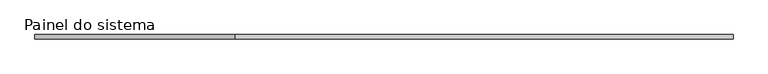
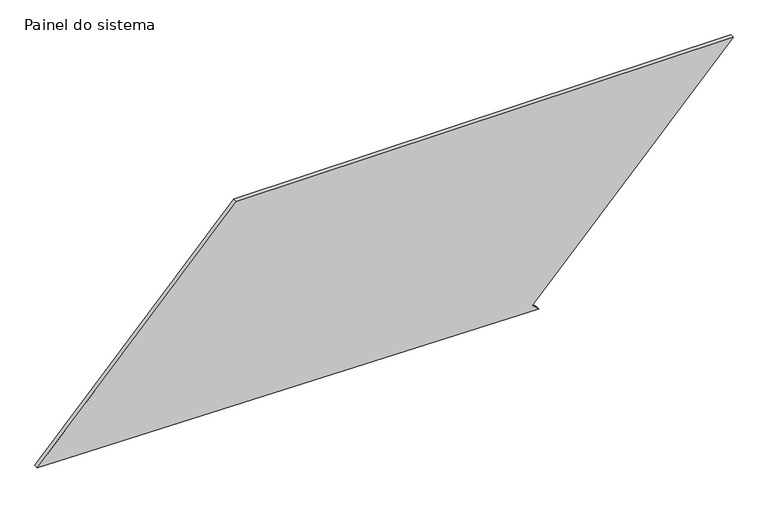
"""IFC4 building model written with IfcOpenShell, lengths in millimetres: plate geometry, Painel do sistema : Envidraçado."""

from ifc_helpers import new_model, si_unit, frame, origin, place, context, project, spatial, polyline, outline, extrude, source, transform, mapped, element, save


def painel_do_sistema_7ac20622(model_context):
    return source(origin(), model_context, "Body", "SweptSolid", [
        extrude(outline(polyline([(0.0, 874.5908783), (34.2393168, 838.1536832), (1251.0437726, 1981.5609368), (1251.0437726, -847.7667432), (44.4694549, -1981.5609368), (0.0, 874.5908783)])), frame((0.0, 24.5, 0.0), z_axis=(0.0, 1.0, 0.0), x_axis=(0.0, 0.0, 1.0)), (0.0, 0.0, 1.0), 25.0),
    ])


if __name__ == "__main__":
    model = new_model("IFC4")
    model_context = context("Model", 3, world=origin())
    ifc_project = project(units=[si_unit("LENGTHUNIT", "METRE", prefix="MILLI")], contexts=[model_context])
    site = spatial("IfcSite", under=ifc_project)
    building = spatial("IfcBuilding", under=site)
    placement = place(None, origin())
    painel_do_sistema_shape = painel_do_sistema_7ac20622(model_context)
    element("IfcPlate", 1, ObjectType="Painel do sistema : Envidraçado", at=placement, inside=building, context=model_context, shape_type="MappedRepresentation", body=[
        mapped(painel_do_sistema_shape, transform((0.0, 0.0, 0.0), x_axis=(1.0, 0.0, 0.0), y_axis=(0.0, 1.0, 0.0), z_axis=(0.0, 0.0, 1.0))),
    ])
    save(model, "model.ifc")

# Revit data of these elements
# Type "Painel do sistema : Envidraçado"
#   Construction Type Id = "GSP4R"
#   Analytic Construction = "Vidraça única Pilkington 1/8 pol"
#   Visual Light Transmittance = 0.9
#   Solar Heat Gain Coefficient = 0.86
#   Heat Transfer Coefficient (U) = 6.7069 W/(m²·K)
# Element 1 (IfcPlate, "Painel do sistema : Envidraçado")
#   Materials on its faces: "Vidro"
# Materials
#   "Vidro": class "Vidro", colour RGB 0 128 192, transparency 0.9, Description = "Vidro de sílica", Cost = 0
